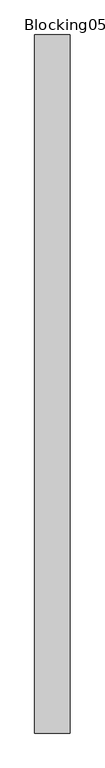
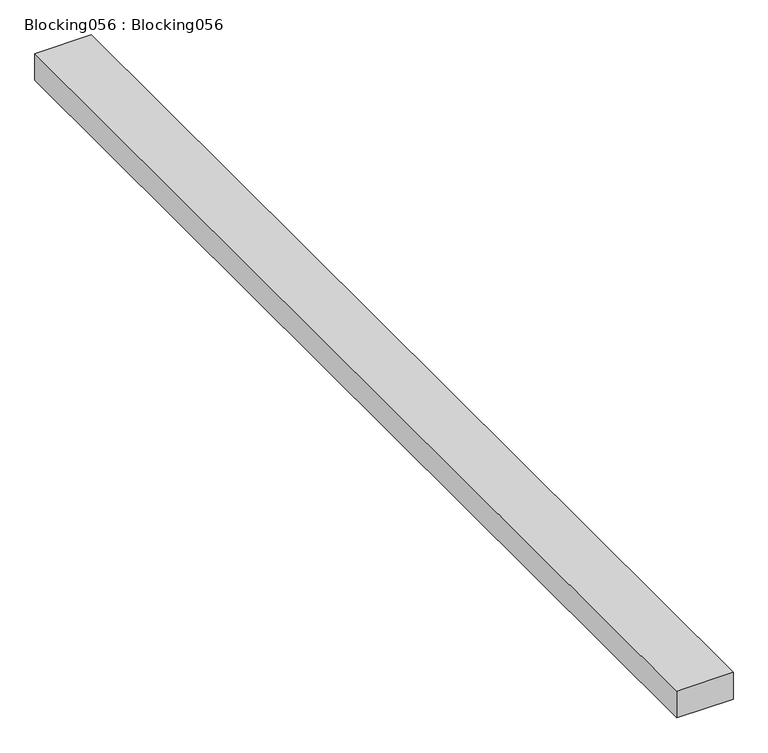
"""IFC4 building model written with IfcOpenShell, lengths in millimetres: proxy geometry, Blocking056 : Blocking056."""

from ifc_helpers import new_model, si_unit, frame, origin, place, context, project, spatial, polyline, outline, extrude, source, transform, mapped, element, save


def blocking056_blocking056_5a466b29(model_context):
    return source(origin(), model_context, "Body", "SweptSolid", [
        extrude(outline(polyline([(-9298.3737014, 7982.1531721), (-9399.9737014, 7982.1531721), (-9399.9737014, 9982.1531721), (-9298.3737014, 9982.1531721), (-9298.3737014, 7982.1531721)])), frame((0.0, 0.0, 40055.5460083), z_axis=(0.0, 0.0, 1.0), x_axis=(1.0, 0.0, 0.0)), (0.0, 0.0, 1.0), 50.8),
    ])


if __name__ == "__main__":
    model = new_model("IFC4")
    model_context = context("Model", 3, world=origin())
    ifc_project = project(units=[si_unit("LENGTHUNIT", "METRE", prefix="MILLI")], contexts=[model_context])
    site = spatial("IfcSite", under=ifc_project)
    building = spatial("IfcBuilding", under=site)
    placement = place(None, origin())
    blocking056_blocking056_shape = blocking056_blocking056_5a466b29(model_context)
    element("IfcBuildingElementProxy", 1, Name="Blocking056 : Blocking056", ObjectType="Blocking056 : Blocking056", at=placement, inside=building, context=model_context, shape_type="MappedRepresentation", body=[
        mapped(blocking056_blocking056_shape, transform((0.0, 0.0, 0.0), x_axis=(1.0, 0.0, 0.0), y_axis=(0.0, 1.0, 0.0), z_axis=(0.0, 0.0, 1.0))),
    ])
    save(model, "model.ifc")

# Revit data of these elements
# Type "Blocking056 : Blocking056"
#   NameOverride = "Blocking056"
# Element 1 (IfcBuildingElementProxy, "Blocking056 : Blocking056")
#   Materials on its faces: "WOOD BLOCKING AS REQUIRED"
# Materials
#   "WOOD BLOCKING AS REQUIRED": class "Unassigned", colour RGB 166 124 85, transparency 0, Cost = 0
